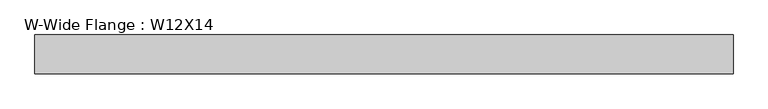
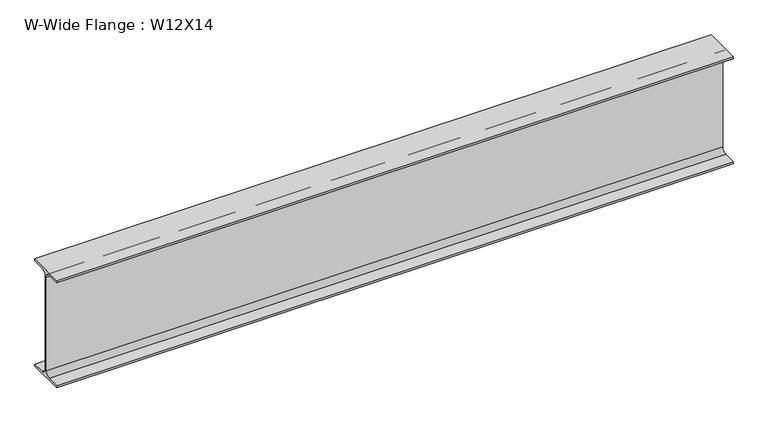
"""IFC4 building model written with IfcOpenShell, lengths in millimetres: beam geometry, W-Wide Flange : W12X14."""

from ifc_helpers import new_model, si_unit, point, frame, frame_2d, origin, place, context, project, spatial, polyline, circle_curve, trimmed, segment, composite_curve, outline, extrude, source, transform, mapped, element, save


def w_wide_flange_w12x14_67c1f98b(model_context):
    return source(origin(), model_context, "Body", "SweptSolid", [
        extrude(outline(composite_curve([segment(polyline([(50.419, -145.415), (50.419, -151.13), (-50.419, -151.13), (-50.419, -145.415), (-15.875, -145.415)]), True, "CONTINUOUS"), segment(trimmed(circle_curve(frame_2d((-15.875, -132.08)), 13.335), [point((-15.875, -145.415))], [point((-2.54, -132.08))], True, "CARTESIAN"), True, "CONTINUOUS"), segment(polyline([(-2.54, -132.08), (-2.54, 132.08)]), True, "CONTINUOUS"), segment(trimmed(circle_curve(frame_2d((-15.875, 132.08)), 13.335), [point((-2.54, 132.08))], [point((-15.875, 145.415))], True, "CARTESIAN"), True, "CONTINUOUS"), segment(polyline([(-15.875, 145.415), (-50.419, 145.415), (-50.419, 151.13), (50.419, 151.13), (50.419, 145.415), (15.875, 145.415)]), True, "CONTINUOUS"), segment(trimmed(circle_curve(frame_2d((15.875, 132.08)), 13.335), [point((15.875, 145.415))], [point((2.54, 132.08))], True, "CARTESIAN"), True, "CONTINUOUS"), segment(polyline([(2.54, 132.08), (2.54, -132.08)]), True, "CONTINUOUS"), segment(trimmed(circle_curve(frame_2d((15.875, -132.08)), 13.335), [point((2.54, -132.08))], [point((15.875, -145.415))], True, "CARTESIAN"), True, "CONTINUOUS"), segment(polyline([(15.875, -145.415), (50.419, -145.415)]), True, "CONTINUOUS")], self_intersect=False)), frame((-915.162, 0.0, 0.0), z_axis=(1.0, 0.0, 0.0), x_axis=(0.0, 1.0, 0.0)), (0.0, 0.0, 1.0), 1804.162),
    ])


if __name__ == "__main__":
    model = new_model("IFC4")
    model_context = context("Model", 3, world=origin())
    ifc_project = project(units=[si_unit("LENGTHUNIT", "METRE", prefix="MILLI")], contexts=[model_context])
    site = spatial("IfcSite", under=ifc_project)
    building = spatial("IfcBuilding", under=site)
    placement = place(None, origin())
    w_wide_flange_w12x14_shape = w_wide_flange_w12x14_67c1f98b(model_context)
    element("IfcBeam", 1, ObjectType="W-Wide Flange : W12X14", at=placement, inside=building, context=model_context, shape_type="MappedRepresentation", body=[
        mapped(w_wide_flange_w12x14_shape, transform((0.0, 0.0, 0.0), x_axis=(1.0, 0.0, 0.0), y_axis=(0.0, 1.0, 0.0), z_axis=(0.0, 0.0, 1.0))),
    ])
    save(model, "model.ifc")

# Revit data of these elements
# Type "W-Wide Flange : W12X14"
#   Assembly Code = "B10"
#   W = 14
#   Length [instance default] = 5' - 0"
#   bf = 0' - 3.97"
#   d = 0' - 11.9"
#   k = 0' - 0 3/4"
#   k2 = 0' - 0.525"
#   tf = 0' - 0.225"
#   tw = 0' - 0.2"
#   A = 0.0288889 SF
#   Structural Material [instance default] = Steel ASTM A992
# Element 1 (IfcBeam, "W-Wide Flange : W12X14")
#   Materials on its faces: "Steel ASTM A992"
# Materials
#   "Steel ASTM A992": class "Metal", colour RGB 199 199 199, transparency 0, Description = "Structural steel 50ksi", Cost = 0
